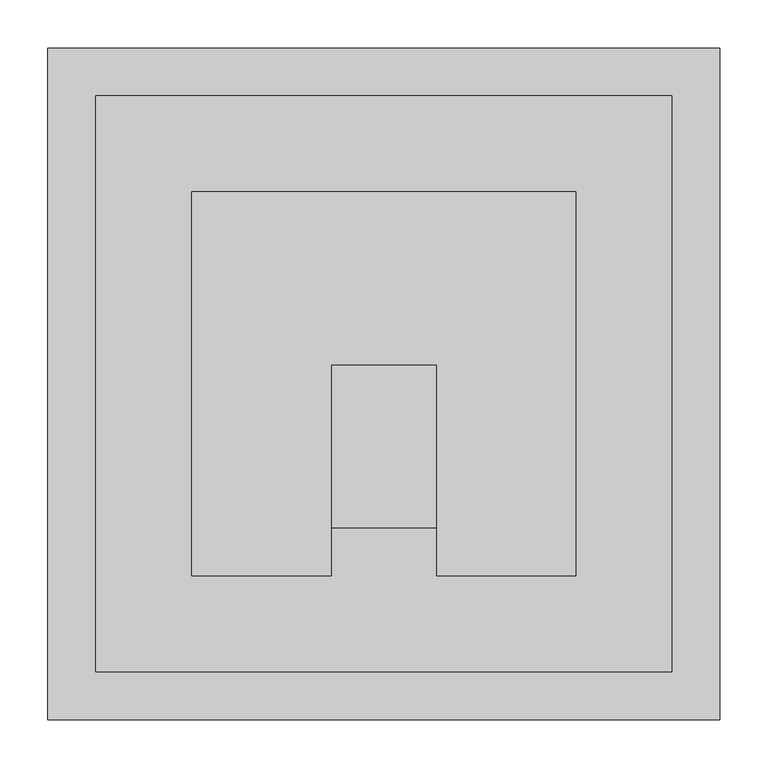
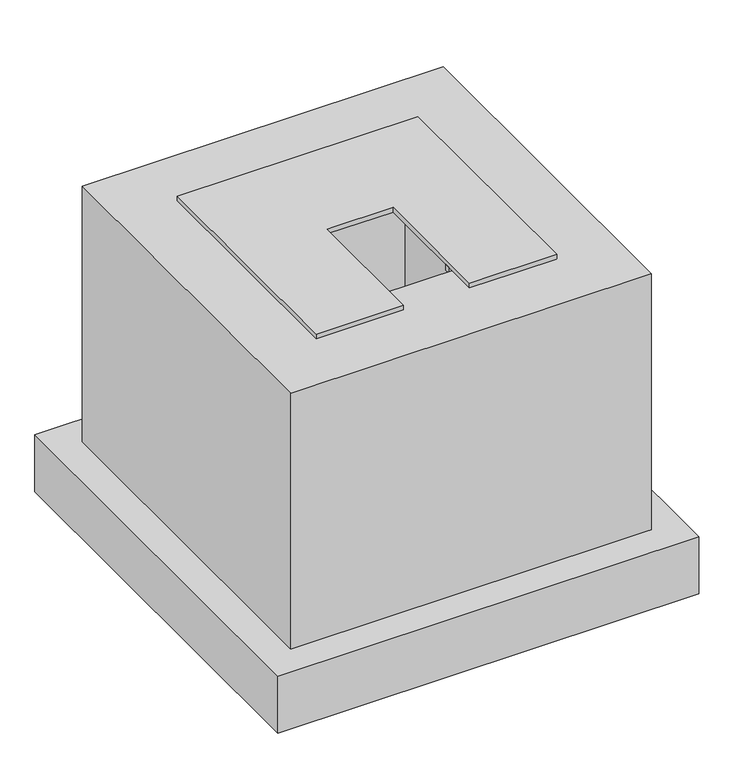
"""IFC4 building model written with IfcOpenShell, lengths in millimetres: proxy geometry, Catchpit : Rainwater Catchpit."""

from ifc_helpers import new_model, si_unit, frame, origin, origin_with_axes, place, context, project, spatial, polyline, outline, extrude, faceted_brep, source, transform, mapped, element, save


def generic_models_1eaa761a(model_context):
    return source(origin(), model_context, "Body", "SolidModel", [
        extrude(outline(polyline([(-55.0, -140.0), (-140.0, -140.0), (-140.0, 140.0), (140.0, 140.0), (140.0, -140.0), (55.0, -140.0), (55.0, -132.0), (132.0, -132.0), (132.0, 132.0), (-132.0, 132.0), (-132.0, -132.0), (-55.0, -132.0), (-55.0, -140.0)])), frame((0.0, 0.0, -10.0), z_axis=(0.0, 0.0, 1.0), x_axis=(1.0, 0.0, 0.0)), (0.0, 0.0, 1.0), 10.0),
        extrude(outline(polyline([(-55.0, -200.0), (-200.0, -200.0), (-200.0, 200.0), (200.0, 200.0), (200.0, -200.0), (55.0, -200.0), (55.0, 20.0), (-55.0, 20.0), (-55.0, -200.0)])), origin_with_axes(), (0.0, 0.0, 1.0), 8.0),
        faceted_brep([(150.0, 150.0, -300.0), (-150.0, 150.0, -300.0), (-150.0, -150.0, -300.0), (150.0, -150.0, -300.0), (300.0, -300.0, -450.0), (-300.0, -300.0, -450.0), (-300.0, 300.0, -450.0), (300.0, 300.0, -450.0), (300.0, -300.0, 0.0), (-300.0, -300.0, 0.0), (-300.0, 300.0, 0.0), (300.0, 300.0, 0.0), (150.0, -150.0, 0.0), (-150.0, -150.0, 0.0), (-150.0, 150.0, 0.0), (150.0, 150.0, 0.0)], [[[0, 1, 2, 3]], [[4, 5, 6, 7]], [[4, 8, 9, 5]], [[9, 10, 6, 5]], [[10, 11, 7, 6]], [[11, 8, 4, 7]], [[8, 11, 10, 9], [12, 13, 14, 15]], [[15, 0, 3, 12]], [[14, 1, 0, 15]], [[13, 2, 1, 14]], [[12, 3, 2, 13]]]),
        extrude(outline(polyline([(350.0, -350.0), (-350.0, -350.0), (-350.0, 350.0), (350.0, 350.0), (350.0, -350.0)])), frame((0.0, 0.0, -550.0), z_axis=(0.0, 0.0, 1.0), x_axis=(1.0, 0.0, 0.0)), (0.0, 0.0, 1.0), 100.0),
    ])


if __name__ == "__main__":
    model = new_model("IFC4")
    model_context = context("Model", 3, world=origin())
    ifc_project = project(units=[si_unit("LENGTHUNIT", "METRE", prefix="MILLI")], contexts=[model_context])
    site = spatial("IfcSite", under=ifc_project)
    building = spatial("IfcBuilding", under=site)
    placement = place(None, origin())
    generic_models_shape = generic_models_1eaa761a(model_context)
    element("IfcBuildingElementProxy", 1, Name="Catchpit : Rainwater Catchpit", ObjectType="Catchpit : Rainwater Catchpit", at=placement, inside=building, context=model_context, shape_type="MappedRepresentation", body=[
        mapped(generic_models_shape, transform((0.0, 0.0, 0.0), x_axis=(1.0, 0.0, 0.0), y_axis=(0.0, 1.0, 0.0), z_axis=(0.0, 0.0, 1.0))),
    ])
    save(model, "model.ifc")

# Revit data of these elements
# Type "Catchpit : Rainwater Catchpit"
#   Width = 300 mm
#   Wall Thk = 150 mm
#   Slab Thk = 150 mm
#   Length = 300 mm
#   Lean Thk = 100 mm
#   Lean Edge = 50 mm
#   Height = 300 mm
#   FB Thk = 8 mm
#   FB Length = 10 mm
#   Cutting Width = 110 mm
#   Cutting Length = 220 mm
#   Chk'd PL Thk = 8 mm
#   Structure Material = none
#   Lean_Material = none
#   CHK`D = none
#   Default Elevation = 0
